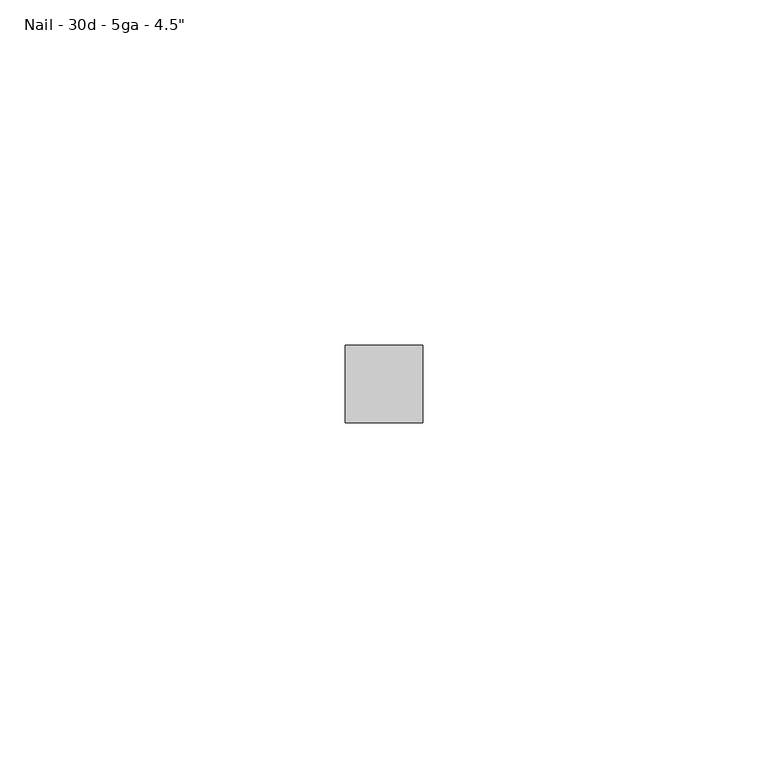
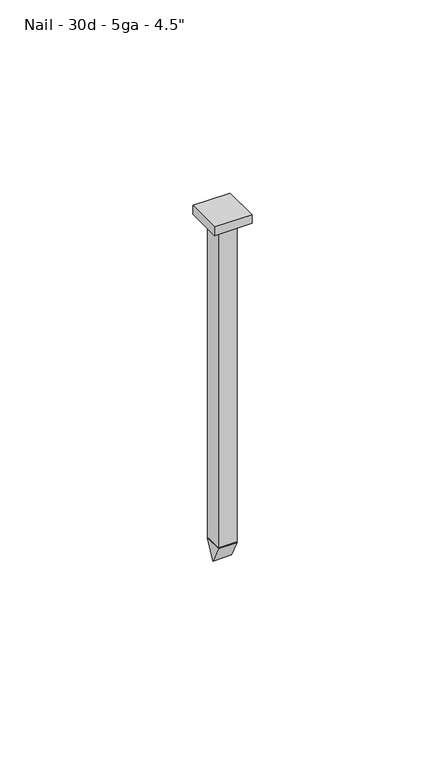
"""IFC4 building model written with IfcOpenShell, lengths in millimetres: fastener geometry."""

from ifc_helpers import new_model, si_unit, frame, origin, origin_with_axes, place, context, project, spatial, polyline, outline, extrude, source, transform, mapped, element, save


def fastener_3e67c611(model_context):
    return source(origin(), model_context, "Body", "SweptSolid", [
        extrude(outline(polyline([(0.0, -107.188), (-2.794, -101.6), (2.794, -101.6), (0.0, -107.188)])), frame((-2.794, 0.0, 0.0), z_axis=(1.0, 0.0, 0.0), x_axis=(0.0, 1.0, 0.0)), (0.0, 0.0, 1.0), 5.588),
        extrude(outline(polyline([(-5.588, -5.588), (-5.588, 5.588), (5.588, 5.588), (5.588, -5.588), (-5.588, -5.588)])), origin_with_axes(), (0.0, 0.0, 1.0), 2.794),
        extrude(outline(polyline([(-2.794, 2.794), (2.794, 2.794), (2.794, -2.794), (-2.794, -2.794), (-2.794, 2.794)])), frame((0.0, 0.0, -101.6), z_axis=(0.0, 0.0, 1.0), x_axis=(1.0, 0.0, 0.0)), (0.0, 0.0, 1.0), 101.6),
    ])


if __name__ == "__main__":
    model = new_model("IFC4")
    model_context = context("Model", 3, world=origin())
    ifc_project = project(units=[si_unit("LENGTHUNIT", "METRE", prefix="MILLI")], contexts=[model_context])
    site = spatial("IfcSite", under=ifc_project)
    building = spatial("IfcBuilding", under=site)
    placement = place(None, origin())
    fastener_shape = fastener_3e67c611(model_context)
    element("IfcFastener", 1, ObjectType="060523 - W_P_C - Fastenings - Generic - SQUARE : Nail - 30d - 5ga - 4.5\"", at=placement, inside=building, context=model_context, shape_type="MappedRepresentation", body=[
        mapped(fastener_shape, transform((0.0, 0.0, 0.0), x_axis=(1.0, 0.0, 0.0), y_axis=(0.0, 1.0, 0.0), z_axis=(0.0, 0.0, 1.0))),
    ])
    save(model, "model.ifc")

# Revit data of these elements
# Type "060523 - W_P_C - Fastenings - Generic - SQUARE : Nail - 30d - 5ga - 4.5\""
#   Washer_Thickness = 0' - 0.00333"
#   Washer Radius = 0' - 0.12"
#   Washer Offset - Head = 0' - 0"
#   Washer Offset = 0' - 0"
#   Thickness_of_Substrate [instance default] = 0' - 1"
#   Side = 0' - 0 37/64"
#   Radius = 0' - 0.11"
#   Length [instance default] = 0' - 4 1/2"
#   Head Size = 0' - 1"
#   Head Radius = 0' - 0 1/2"
#   Head Height = 0' - 0.01"
#   Double Diameter = 0' - 0.44"
#   Diameter = 0' - 0.22"
#   Default Elevation = 4' - 0"
#   Washer_Nut_Visibility = no
#   Washer_Head_Visibility = no
#   Round_Head_Visibility = yes
#   Point Visibility = yes
#   Nut_Visibility = no
#   Hex_Head_Visiblilty = no
#   Washer Material = none
#   Bolt Material (Size) = AT SILL - FASTENER AT 24" O.C.
# Element 1 (IfcFastener, "060523 - W_P_C - Fastenings - Generic - SQUARE : Nail - 30d - 5ga - 4.5\"")
#   Length = 0' - 4"
# Materials
#   "AT SILL - FASTENER AT 24\" O.C.": class "Generic", colour RGB 120 120 120, transparency 0, Cost = 0
